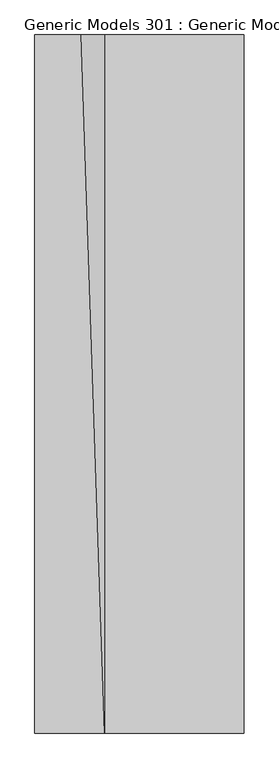
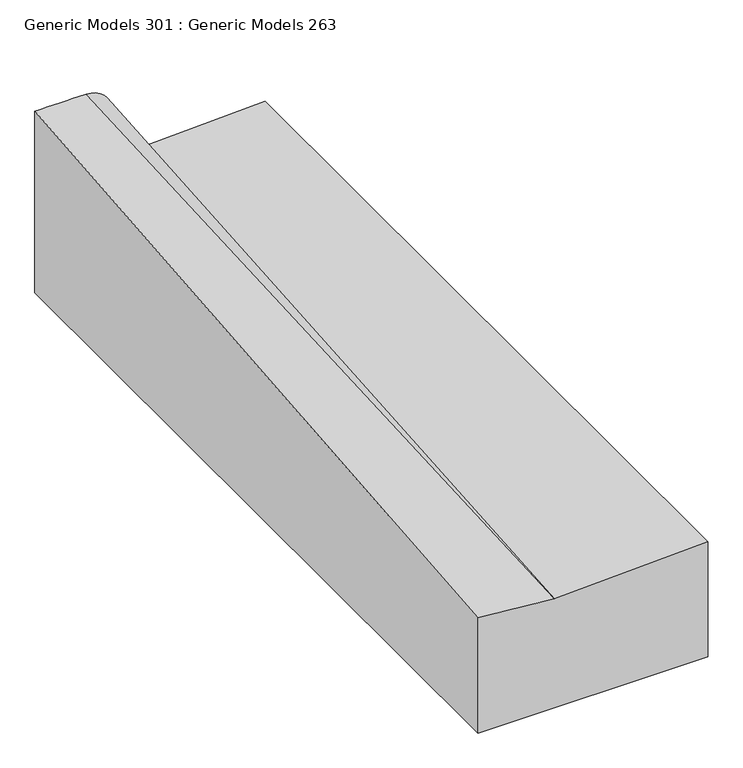
"""IFC4 building model written with IfcOpenShell, lengths in millimetres: proxy geometry, Generic Models 301 : Generic Models 263."""

from ifc_helpers import new_model, si_unit, frame, origin, place, context, project, spatial, circle_curve, source, transform, mapped, element, save
from ifc_brep_helpers import plane_surface, spline_surface, advanced_brep


def generic_models_301_generic_models_263_c6164b38(model_context):
    return source(origin(), model_context, "Body", "AdvancedBrep", [
        advanced_brep(
        [(91579.9797726, 582.5727422, -139.1379392), (91579.9797726, 582.5727422, -381.0), (92037.1797726, 582.5727422, -381.0), (92037.1797726, 582.5727422, -139.7), (91732.3797726, 582.5727422, -152.4), (91579.9797726, 2106.5727422, 0.0), (91681.5797726, 2106.5727422, 0.0), (91732.3797726, 2106.5727422, -50.8), (91732.3797726, 2106.5727422, -152.4), (92037.1797726, 2106.5727422, -139.7), (92037.1797726, 2106.5727422, -381.0), (91579.9797726, 2106.5727422, -381.0)],
        [
            (0, 1),
            (1, 2),
            (2, 3),
            (3, 4),
            (4, 0),
            (5, 6),
            (6, 7, circle_curve(frame((91681.5797726, 2106.5727422, -50.8), z_axis=(0.0, 1.0, 0.0), x_axis=(1.0, 0.0, 0.0)), 50.8)),
            (7, 8),
            (8, 9),
            (9, 10),
            (10, 11),
            (11, 5),
            (11, 1),
            (0, 5),
            (10, 2),
            (9, 3),
            (7, 4),
            (4, 8),
            (6, 4),
        ],
        [
            plane_surface(frame((91793.3397726, 582.5727422, -238.6475878), z_axis=(0.0, -1.0, 0.0), x_axis=(1.0, 0.0, 0.0))),
            plane_surface(frame((91768.6654869, 2106.5727422, -157.8428571), z_axis=(0.0, 1.0, 0.0), x_axis=(1.0, 0.0, 0.0))),
            plane_surface(frame((91579.9797726, 2106.5727422, -190.5), z_axis=(-1.0, 0.0, 0.0), x_axis=(0.0, 0.0, -1.0))),
            plane_surface(frame((91808.5797726, 2106.5727422, -381.0), z_axis=(0.0, 0.0, -1.0), x_axis=(1.0, 0.0, 0.0))),
            plane_surface(frame((92037.1797726, 2106.5727422, -260.35), z_axis=(1.0, 0.0, 0.0), x_axis=(0.0, 0.0, 1.0))),
            plane_surface(frame((91732.3797726, 2106.5727422, -101.6), z_axis=(1.0, 0.0, 0.0), x_axis=(0.0, 0.0, 1.0))),
            spline_surface(2, 1, [[(91732.3797726, 2106.5727422, -50.8), (91732.3797726, 582.5727422, -152.4)], [(91732.3797726, 2106.5727422, 2.9132252166164108e-12), (91732.3797726, 582.5727422, -152.4)], [(91681.5797726, 2106.5727422, 0.0), (91732.3797726, 582.5727422, -152.4)]], [3, 3], [2, 2], [0.0, 1.0], [0.0, 1.0], weights=[[1.0, 1.0], [0.7071067811865273, 0.7071067811865273], [1.0, 1.0]]),
            spline_surface(1, 1, [[(91681.5797726, 2106.5727422, 0.0), (91732.3797726, 582.5727422, -152.4)], [(91579.9797726, 2106.5727422, 0.0), (91579.9797726, 582.5727422, -139.1379392)]], [2, 2], [2, 2], [0.0, 1.0], [0.0, 1.0]),
            plane_surface(frame((91884.7797726, 2106.5727422, -146.05), z_axis=(-0.04163054471218724, 0.0, 0.9991330730923517), x_axis=(-0.9991330730923517, 0.0, -0.04163054471218724))),
        ],
        [
            (0, [[1, 2, 3, 4, 5]]),
            (1, [[6, 7, 8, 9, 10, 11, 12]]),
            (2, [[-12, 13, -1, 14]]),
            (3, [[-11, 15, -2, -13]]),
            (4, [[-10, 16, -3, -15]]),
            (5, [[-8, 17, 18]]),
            (6, [[-7, 19, -17]]),
            (7, [[-6, -14, -5, -19]]),
            (8, [[-9, -18, -4, -16]]),
        ],
    ),
    ])


if __name__ == "__main__":
    model = new_model("IFC4")
    model_context = context("Model", 3, world=origin())
    ifc_project = project(units=[si_unit("LENGTHUNIT", "METRE", prefix="MILLI")], contexts=[model_context])
    site = spatial("IfcSite", under=ifc_project)
    building = spatial("IfcBuilding", under=site)
    placement = place(None, origin())
    generic_models_301_generic_models_263_shape = generic_models_301_generic_models_263_c6164b38(model_context)
    element("IfcBuildingElementProxy", 1, Name="Generic Models 301 : Generic Models 263", ObjectType="Generic Models 301 : Generic Models 263", at=placement, inside=building, context=model_context, shape_type="MappedRepresentation", body=[
        mapped(generic_models_301_generic_models_263_shape, transform((0.0, 0.0, 0.0), x_axis=(1.0, 0.0, 0.0), y_axis=(0.0, 1.0, 0.0), z_axis=(0.0, 0.0, 1.0))),
    ])
    save(model, "model.ifc")

# Revit data of these elements
# Element 1 (IfcBuildingElementProxy, "Generic Models 301 : Generic Models 263")
#   Materials on its faces: "CONCRETE CURB"
# Materials
#   "CONCRETE CURB": class "Concrete", colour RGB 191 191 191, transparency 0, Description = "Cast-in-place concrete", Cost = 0
